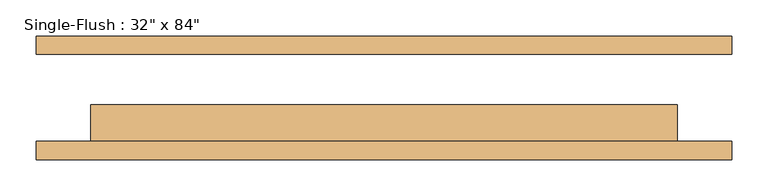
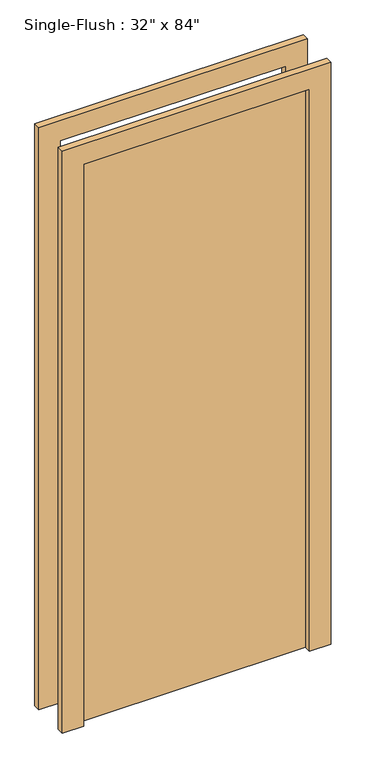
"""IFC4 building model written with IfcOpenShell, lengths in millimetres: door geometry."""

from ifc_helpers import new_model, si_unit, frame, origin, origin_with_axes, place, context, project, spatial, polyline, outline, extrude, source, transform, mapped, element, save


def door_40fd8627(model_context):
    return source(origin(), model_context, "Body", "SweptSolid", [
        extrude(outline(polyline([(2209.8, -482.6), (0.0, -482.6), (0.0, -406.4), (2133.6, -406.4), (2133.6, 406.4), (0.0, 406.4), (0.0, 482.6), (2209.8, 482.6), (2209.8, -482.6)])), frame((0.0, -85.725, 0.0), z_axis=(0.0, 1.0, 0.0), x_axis=(0.0, 0.0, 1.0)), (0.0, 0.0, 1.0), 25.4),
        extrude(outline(polyline([(2209.8, 482.6), (2209.8, -482.6), (0.0, -482.6), (0.0, -406.4), (2133.6, -406.4), (2133.6, 406.4), (0.0, 406.4), (0.0, 482.6), (2209.8, 482.6)])), frame((0.0, 60.325, 0.0), z_axis=(0.0, 1.0, 0.0), x_axis=(0.0, 0.0, 1.0)), (0.0, 0.0, 1.0), 25.4),
        extrude(outline(polyline([(406.4, -9.525), (406.4, -60.325), (-406.4, -60.325), (-406.4, -9.525), (406.4, -9.525)])), origin_with_axes(), (0.0, 0.0, 1.0), 2133.6),
    ])


if __name__ == "__main__":
    model = new_model("IFC4")
    model_context = context("Model", 3, world=origin())
    ifc_project = project(units=[si_unit("LENGTHUNIT", "METRE", prefix="MILLI")], contexts=[model_context])
    site = spatial("IfcSite", under=ifc_project)
    building = spatial("IfcBuilding", under=site)
    placement = place(None, origin())
    door_shape = door_40fd8627(model_context)
    element("IfcDoor", 1, ObjectType="Single-Flush : 32\" x 84\"", at=placement, inside=building, context=model_context, shape_type="MappedRepresentation", body=[
        mapped(door_shape, transform((0.0, 0.0, 0.0), x_axis=(1.0, 0.0, 0.0), y_axis=(0.0, 1.0, 0.0), z_axis=(0.0, 0.0, 1.0))),
    ])
    save(model, "model.ifc")

# Revit data of these elements
# Type "Single-Flush : 32\" x 84\""
#   Type Mark = "10"
#   Construction Type Id = "MDOOR"
#   Assembly Code = "C1020"
#   Analytic Construction = "Metal"
#   Thickness = 0' - 2"
#   Heat Transfer Coefficient (U) = 3.7021 W/(m²·K)
#   Height = 7' - 0"
#   Trim Projection Ext = 0' - 1"
#   Trim Projection Int = 0' - 1"
#   Trim Width = 0' - 3"
#   Width = 2' - 8"
#   Door Material = Door - Panel
#   Frame Material = Door - Frame
#   Visual Light Transmittance = 0
#   Solar Heat Gain Coefficient = 0
#   Function = (empty or 0)
#   Wall Closure = (empty or 0)
# Element 1 (IfcDoor, "Single-Flush : 32\" x 84\"")
#   Materials on its faces: "Door - Frame", "Door - Panel"
# Materials
#   "Door - Panel": class "Wood", colour RGB 210 159 95, transparency 0
#   "Door - Frame": class "Miscellaneous", colour RGB 118 70 51, transparency 0
